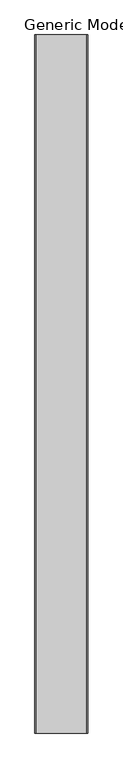
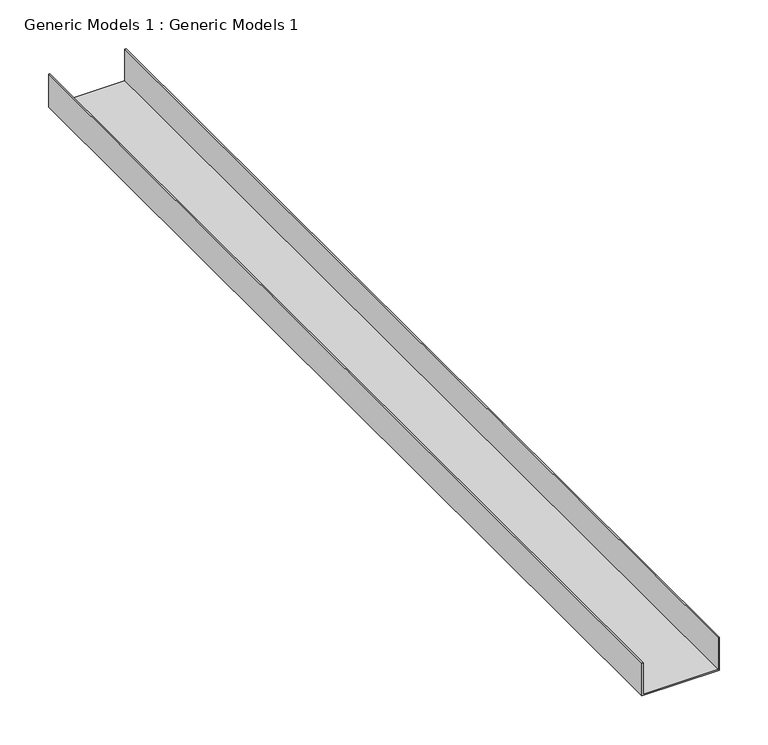
"""IFC4 building model written with IfcOpenShell, lengths in millimetres: proxy geometry, Generic Models 1 : Generic Models 1."""

import ifcopenshell
import ifcopenshell.guid

model = None  # the IFC model being written
_history = None  # IfcOwnerHistory: only IFC2X3 demands one
_inside = {}  # id of a spatial element -> (the spatial element, [elements in it])
_under = {}  # id of a project, library or spatial element -> (it, [spatial elements below it])
_declared = {}  # id of a project -> (the project, [libraries it declares])
_typed = {}  # id of a type object -> (the type object, [elements of that type])
_made_of = {}  # id of a material, layer set ... -> (it, [elements and type objects made of it])


def new_model(schema):
    """Start an empty IFC model of exactly this schema.

    Asked for "IFC4X3", IfcOpenShell would pick the latest addendum, in which some entities
    have other attributes; the version numbers below select the first issue.
    IFC2X3 requires an IfcOwnerHistory on every rooted entity: one is made here for all.
    """
    global model, _history
    if schema == "IFC4X3":
        model = ifcopenshell.file(schema_version=(4, 3, 0, 0))
    else:
        model = ifcopenshell.file(schema=schema)
    _inside.clear()
    _under.clear()
    _declared.clear()
    _typed.clear()
    _made_of.clear()
    _history = None
    if model.schema == "IFC2X3":
        org = make("IfcOrganization", Name="unknown")
        user = make(
            "IfcPersonAndOrganization",
            ThePerson=make("IfcPerson", FamilyName="unknown"),
            TheOrganization=org,
        )
        app = make(
            "IfcApplication",
            ApplicationDeveloper=org,
            Version="unknown",
            ApplicationFullName="unknown",
            ApplicationIdentifier="unknown",
        )
        _history = make(
            "IfcOwnerHistory",
            OwningUser=user,
            OwningApplication=app,
            ChangeAction="ADDED",
            CreationDate=0,
        )
    return model


def make(cls, **values):
    """One entity of the class cls with the attributes given. An attribute that is None is left unset."""
    return model.create_entity(
        cls, **{name: value for name, value in values.items() if value is not None}
    )


def rooted(cls, **values):
    """An entity with a GlobalId (a new one), such as an element, a storey or a relation."""
    return make(cls, GlobalId=ifcopenshell.guid.new(), OwnerHistory=_history, **values)


def si_unit(unit_type, name, prefix=None):
    """IfcSIUnit, for example si_unit("LENGTHUNIT", "METRE", prefix="MILLI")."""
    return make("IfcSIUnit", UnitType=unit_type, Prefix=prefix, Name=name)


def assignment(units):
    """IfcUnitAssignment: the units of a project."""
    return None if units is None else make("IfcUnitAssignment", Units=units)


def point(xyz):
    """IfcCartesianPoint."""
    return None if xyz is None else make("IfcCartesianPoint", Coordinates=xyz)


def direction(xyz):
    """IfcDirection."""
    return None if xyz is None else make("IfcDirection", DirectionRatios=xyz)


def frame(location, z_axis=None, x_axis=None):
    """IfcAxis2Placement3D, a coordinate frame: its origin and axes. An axis left out is left unset."""
    return make(
        "IfcAxis2Placement3D",
        Location=point(location),
        Axis=direction(z_axis),
        RefDirection=direction(x_axis),
    )


def origin():
    """The frame at (0, 0, 0) with its axes left unset."""
    return frame((0.0, 0.0, 0.0))


def place(relative_to, where):
    """IfcLocalPlacement: puts the frame where relative to a parent placement (None: the world)."""
    return make(
        "IfcLocalPlacement", PlacementRelTo=relative_to, RelativePlacement=where
    )


def context(
    kind, dimensions, precision=None, world=None, true_north=None, identifier=None
):
    """IfcGeometricRepresentationContext, for example the 3D "Model" context."""
    return make(
        "IfcGeometricRepresentationContext",
        ContextIdentifier=identifier,
        ContextType=kind,
        CoordinateSpaceDimension=dimensions,
        Precision=precision,
        WorldCoordinateSystem=world,
        TrueNorth=true_north,
    )


def project(units=None, contexts=None):
    """IfcProject with its units and contexts."""
    return rooted(
        "IfcProject",
        Name="project",
        RepresentationContexts=contexts,
        UnitsInContext=assignment(units),
    )


def spatial(cls, under=None, at=None, **own):
    """A site, building, storey or space (cls), placed at a placement, below another one or the project."""
    s = rooted(cls, ObjectPlacement=at, **own)
    if under is not None:
        _under.setdefault(under.id(), (under, []))[1].append(s)
    return s


def polyline(points):
    """IfcPolyline through the points."""
    return make("IfcPolyline", Points=[point(p) for p in points])


def outline(outer, holes=None, kind="AREA"):
    """IfcArbitraryClosedProfileDef: a profile drawn as a closed curve; with holes, ...WithVoids."""
    if holes is None:
        return make("IfcArbitraryClosedProfileDef", ProfileType=kind, OuterCurve=outer)
    return make(
        "IfcArbitraryProfileDefWithVoids",
        ProfileType=kind,
        OuterCurve=outer,
        InnerCurves=holes,
    )


def extrude(swept, where, along, depth):
    """IfcExtrudedAreaSolid: the profile swept, set in the frame where, extruded along a direction by depth."""
    return make(
        "IfcExtrudedAreaSolid",
        SweptArea=swept,
        Position=where,
        ExtrudedDirection=direction(along),
        Depth=depth,
    )


def shape(context_of_items, identifier, shape_type, items):
    """IfcShapeRepresentation: the items that make up one representation, for example the "Body"."""
    return make(
        "IfcShapeRepresentation",
        ContextOfItems=context_of_items,
        RepresentationIdentifier=identifier,
        RepresentationType=shape_type,
        Items=items,
    )


def source(mapping_origin, context_of_items, identifier, shape_type, items):
    """IfcRepresentationMap: a shape defined once, which mapped items show again and again."""
    return make(
        "IfcRepresentationMap",
        MappingOrigin=mapping_origin,
        MappedRepresentation=shape(context_of_items, identifier, shape_type, items),
    )


def transform(
    local_origin,
    x_axis=None,
    y_axis=None,
    z_axis=None,
    scale=None,
    scale2=None,
    scale3=None,
    uniform=True,
):
    """IfcCartesianTransformationOperator3D, or its non-uniform kind. x_axis, y_axis, z_axis: its Axis1, 2, 3."""
    if uniform:
        return make(
            "IfcCartesianTransformationOperator3D",
            Axis1=direction(x_axis),
            Axis2=direction(y_axis),
            LocalOrigin=point(local_origin),
            Scale=scale,
            Axis3=direction(z_axis),
        )
    return make(
        "IfcCartesianTransformationOperator3DnonUniform",
        Axis1=direction(x_axis),
        Axis2=direction(y_axis),
        LocalOrigin=point(local_origin),
        Scale=scale,
        Axis3=direction(z_axis),
        Scale2=scale2,
        Scale3=scale3,
    )


def mapped(mapping_source, mapping_target):
    """IfcMappedItem: shows the shape of a source again, moved by a transform."""
    return make(
        "IfcMappedItem", MappingSource=mapping_source, MappingTarget=mapping_target
    )


def made_of(thing, what):
    """Note that an element or type object is made of a material, layer set ...; save() writes the relation."""
    if what is not None:
        _made_of.setdefault(what.id(), (what, []))[1].append(thing)
    return thing


def element(
    cls,
    number,
    at=None,
    inside=None,
    cuts=None,
    type_object=None,
    material=None,
    context=None,
    identifier="Body",
    shape_type=None,
    held_by="IfcProductDefinitionShape",
    body=None,
    shapes=None,
    **own,
):
    """One element of the class cls, such as IfcWall. Its Tag is "e" and its number.

    at: its placement. inside: the storey or other place that contains it. cuts: it is an
    opening in that element (IfcRelVoidsElement). A single representation is given by context,
    identifier, shape_type and body (its items); several are given by shapes. held_by: the class
    of the entity that holds the representations. save() writes the other relations.
    """
    e = rooted(cls, Tag="e%d" % number, ObjectPlacement=at, **own)
    if body is not None:
        shapes = [shape(context, identifier, shape_type, body)]
    if shapes is not None:
        e.Representation = make(held_by, Representations=shapes)
    if inside is not None:
        _inside.setdefault(inside.id(), (inside, []))[1].append(e)
    if cuts is not None:
        rooted(
            "IfcRelVoidsElement", RelatingBuildingElement=cuts, RelatedOpeningElement=e
        )
    if type_object is not None:
        _typed.setdefault(type_object.id(), (type_object, []))[1].append(e)
    return made_of(e, material)


def aggregate(whole, parts):
    """IfcRelAggregates: a whole, such as a stair, and the parts it consists of."""
    return rooted("IfcRelAggregates", RelatingObject=whole, RelatedObjects=parts)


def save(model, path):
    """Write the relations noted so far, then the file.

    IfcRelAggregates (storeys below a building ...), IfcRelContainedInSpatialStructure (elements
    in a storey), IfcRelDefinesByType, IfcRelAssociatesMaterial and IfcRelDeclares: one each for
    every whole, place, type object, material and project.
    """
    for whole, parts in _under.values():
        aggregate(whole, parts)
    for where, things in _inside.values():
        rooted(
            "IfcRelContainedInSpatialStructure",
            RelatedElements=things,
            RelatingStructure=where,
        )
    for kind, things in _typed.values():
        rooted("IfcRelDefinesByType", RelatedObjects=things, RelatingType=kind)
    for what, things in _made_of.values():
        rooted("IfcRelAssociatesMaterial", RelatedObjects=things, RelatingMaterial=what)
    for by, libraries in _declared.values():
        rooted("IfcRelDeclares", RelatingContext=by, RelatedDefinitions=libraries)
    model.write(path)


def generic_models_1_generic_models_1_e7a28f78(model_context):
    return source(origin(), model_context, "Body", "SweptSolid", [
        extrude(outline(polyline([(0.0, 51003.2), (41.275, 51003.2), (41.275, 51001.6125), (1.5875, 51001.6125), (1.5875, 50912.7125), (41.275, 50912.7125), (41.275, 50911.125), (0.0, 50911.125), (0.0, 51003.2)])), frame((0.0, 0.0, 0.0), z_axis=(0.0, 1.0, 0.0), x_axis=(0.0, 0.0, 1.0)), (0.0, 0.0, 1.0), 1219.2),
    ])


if __name__ == "__main__":
    model = new_model("IFC4")
    model_context = context("Model", 3, world=origin())
    ifc_project = project(units=[si_unit("LENGTHUNIT", "METRE", prefix="MILLI")], contexts=[model_context])
    site = spatial("IfcSite", under=ifc_project)
    building = spatial("IfcBuilding", under=site)
    placement = place(None, origin())
    generic_models_1_generic_models_1_shape = generic_models_1_generic_models_1_e7a28f78(model_context)
    element("IfcBuildingElementProxy", 1, Name="Generic Models 1 : Generic Models 1", ObjectType="Generic Models 1 : Generic Models 1", at=placement, inside=building, context=model_context, shape_type="MappedRepresentation", body=[
        mapped(generic_models_1_generic_models_1_shape, transform((0.0, 0.0, 0.0), x_axis=(1.0, 0.0, 0.0), y_axis=(0.0, 1.0, 0.0), z_axis=(0.0, 0.0, 1.0))),
    ])
    save(model, "model.ifc")

# Revit data of these elements
# Element 1 (IfcBuildingElementProxy, "Generic Models 1 : Generic Models 1")
#   Materials on its faces: "METAL RUNNER ANCHORED TO STRUCTURE"
# Materials
#   "METAL RUNNER ANCHORED TO STRUCTURE": class "Unassigned", colour RGB 210 209 208, transparency 0, Keynote = "M05121300.02", Cost = 0
